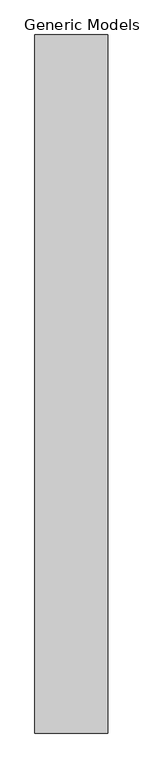
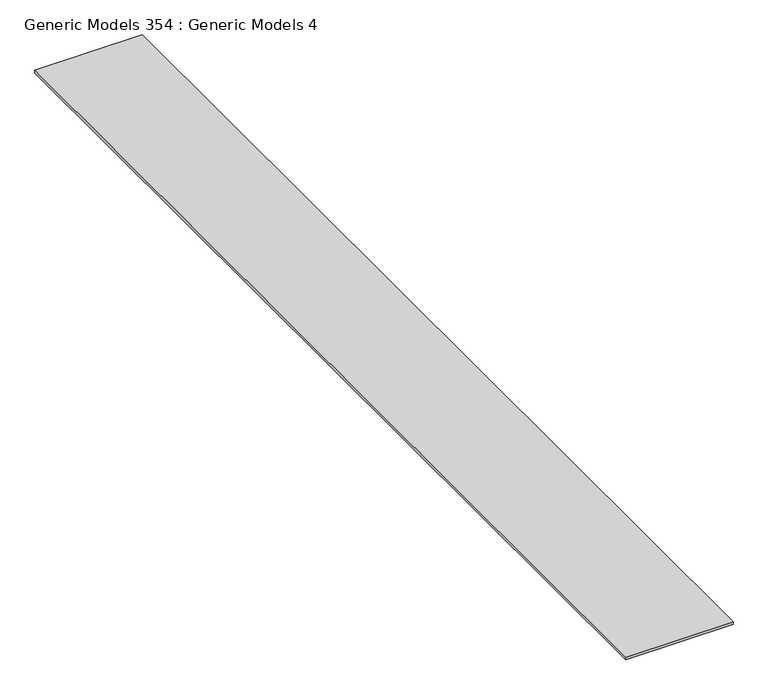
"""IFC4 building model written with IfcOpenShell, lengths in millimetres: proxy geometry, Generic Models 354 : Generic Models 4."""

from ifc_helpers import new_model, si_unit, frame, origin, place, context, project, spatial, polyline, outline, extrude, source, transform, mapped, element, save


def generic_models_354_generic_models_4_cf566790(model_context):
    return source(origin(), model_context, "Body", "SweptSolid", [
        extrude(outline(polyline([(10201.955181, -6864.9230338), (9532.1363263, -6864.9230338), (9532.1363263, -464.1230338), (10201.955181, -464.1230338), (10201.955181, -6864.9230338)])), frame((0.0, 0.0, 126524.8520404), z_axis=(0.0, 0.0, 1.0), x_axis=(1.0, 0.0, 0.0)), (0.0, 0.0, 1.0), 19.05),
    ])


if __name__ == "__main__":
    model = new_model("IFC4")
    model_context = context("Model", 3, world=origin())
    ifc_project = project(units=[si_unit("LENGTHUNIT", "METRE", prefix="MILLI")], contexts=[model_context])
    site = spatial("IfcSite", under=ifc_project)
    building = spatial("IfcBuilding", under=site)
    placement = place(None, origin())
    generic_models_354_generic_models_4_shape = generic_models_354_generic_models_4_cf566790(model_context)
    element("IfcBuildingElementProxy", 1, Name="Generic Models 354 : Generic Models 4", ObjectType="Generic Models 354 : Generic Models 4", at=placement, inside=building, context=model_context, shape_type="MappedRepresentation", body=[
        mapped(generic_models_354_generic_models_4_shape, transform((0.0, 0.0, 0.0), x_axis=(1.0, 0.0, 0.0), y_axis=(0.0, 1.0, 0.0), z_axis=(0.0, 0.0, 1.0))),
    ])
    save(model, "model.ifc")

# Revit data of these elements
# Element 1 (IfcBuildingElementProxy, "Generic Models 354 : Generic Models 4")
#   Materials on its faces: "_CDX PLYWOOD - SEE STRUCT DWGs"
# Materials
#   "_CDX PLYWOOD - SEE STRUCT DWGs": class "Generic", colour RGB 98 75 74, transparency 0, Cost = 0
